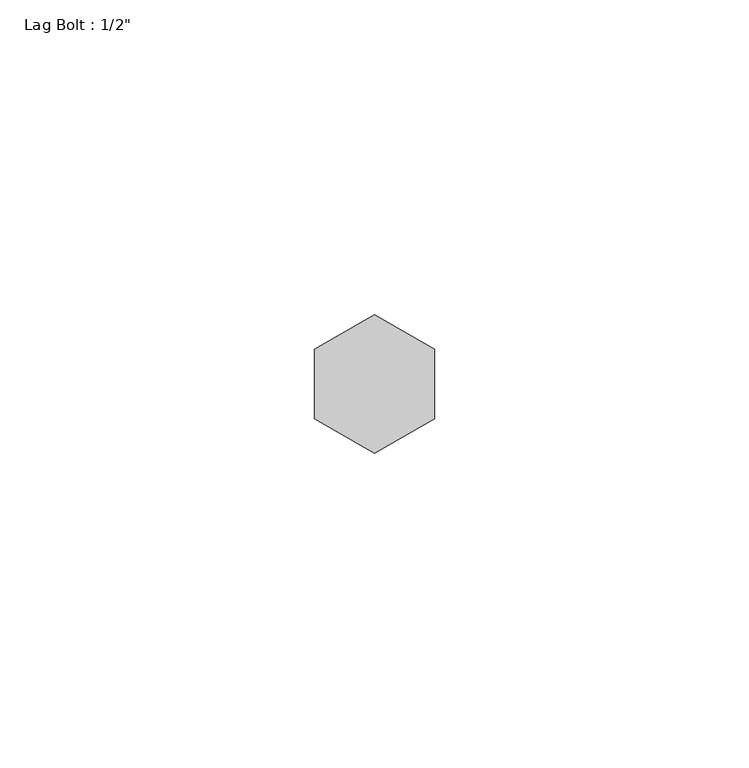
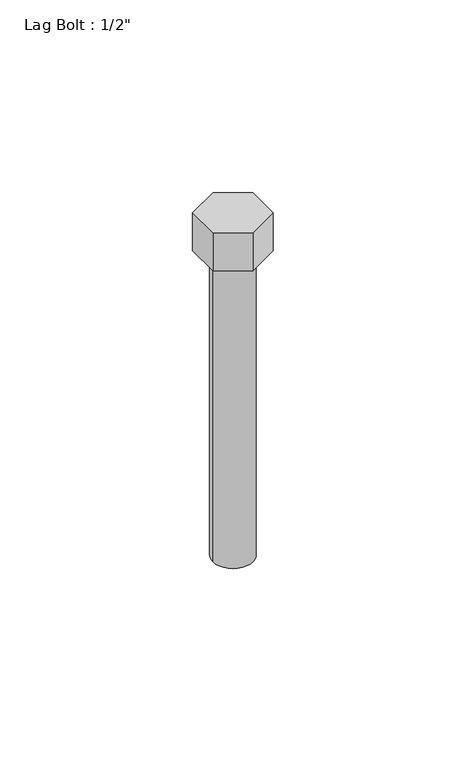
"""IFC4 building model written with IfcOpenShell, lengths in millimetres: proxy geometry."""

from ifc_helpers import new_model, si_unit, point, frame, origin, origin_with_axes, origin_2d, place, context, project, spatial, polyline, circle_curve, trimmed, segment, composite_curve, outline, extrude, source, transform, mapped, element, save


def proxy_7df0dc6f(model_context):
    return source(origin(), model_context, "Body", "SweptSolid", [
        extrude(outline(polyline([(-9.525, 5.4992613), (0.0, 10.9985226), (9.525, 5.4992613), (9.525, -5.4992613), (0.0, -10.9985226), (-9.525, -5.4992613), (-9.525, 5.4992613)])), origin_with_axes(), (0.0, 0.0, 1.0), 12.7),
        extrude(outline(composite_curve([segment(trimmed(circle_curve(origin_2d(), 6.35), [point((-6.35, 0.0))], [point((6.35, 0.0))], False, "CARTESIAN"), True, "CONTINUOUS"), segment(trimmed(circle_curve(origin_2d(), 6.35), [point((6.35, 0.0))], [point((-6.35, 0.0))], False, "CARTESIAN"), True, "CONTINUOUS")], self_intersect=False)), frame((0.0, 0.0, -101.6), z_axis=(0.0, 0.0, 1.0), x_axis=(1.0, 0.0, 0.0)), (0.0, 0.0, 1.0), 101.6),
    ])


if __name__ == "__main__":
    model = new_model("IFC4")
    model_context = context("Model", 3, world=origin())
    ifc_project = project(units=[si_unit("LENGTHUNIT", "METRE", prefix="MILLI")], contexts=[model_context])
    site = spatial("IfcSite", under=ifc_project)
    building = spatial("IfcBuilding", under=site)
    placement = place(None, origin())
    proxy_shape = proxy_7df0dc6f(model_context)
    element("IfcBuildingElementProxy", 1, Name="Lag Bolt : 1/2\"", ObjectType="Lag Bolt : 1/2\"", at=placement, inside=building, context=model_context, shape_type="MappedRepresentation", body=[
        mapped(proxy_shape, transform((0.0, 0.0, 0.0), x_axis=(1.0, 0.0, 0.0), y_axis=(0.0, 1.0, 0.0), z_axis=(0.0, 0.0, 1.0))),
    ])
    save(model, "model.ifc")

# Revit data of these elements
# Type "Lag Bolt : 1/2\""
#   Thickness_of_Substrate [instance default] = 0' - 1"
#   Side = 0' - 0 111/256"
#   Radius = 0' - 0 1/4"
#   Length = 0' - 4"
#   Head Size = 0' - 0 3/4"
#   Head Radius = 0' - 0 3/8"
#   Head Height = 0' - 0 1/2"
#   Diameter = 0' - 0 1/2"
#   Default Elevation = 4' - 0"
#   Nut_Visibility [instance default] = yes
#   Bolt Material (Size) [instance default] = 1/2" X 5" LAG BOLT (THRU BOLT IF PLATE ON OPP. SIDE OF STRUCT MEMBER)
# Element 1 (IfcBuildingElementProxy, "Lag Bolt : 1/2\"")
#   Thickness_of_Substrate = 0' - 4"
#   Nut_Visibility = no
#   Bolt Material (Size) = 1/2" LAG BOLT
#   Materials on its faces: "1/2\" LAG BOLT"
# Materials
#   "1/2\" X 5\" LAG BOLT (THRU BOLT IF PLATE ON OPP. SIDE OF STRUCT MEMBER)": class "Generic", colour RGB 120 120 120, transparency 0, Cost = 0
#   "1/2\" LAG BOLT": class "Generic", colour RGB 120 120 120, transparency 0, Cost = 0
